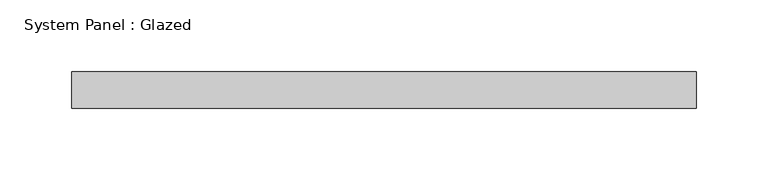
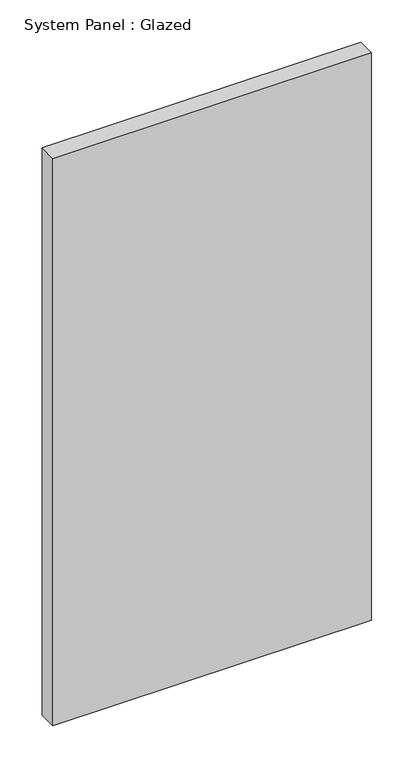
"""IFC4 building model written with IfcOpenShell, lengths in millimetres: plate geometry, System Panel : Glazed."""

from ifc_helpers import new_model, si_unit, origin, origin_with_axes, place, context, project, spatial, polyline, outline, extrude, source, transform, mapped, element, save


def system_panel_glazed_eab43fe1(model_context):
    return source(origin(), model_context, "Body", "SweptSolid", [
        extrude(outline(polyline([(217.839047, 19.05), (-217.839047, 19.05), (-217.839047, 44.45), (217.839047, 44.45), (217.839047, 19.05)])), origin_with_axes(), (0.0, 0.0, 1.0), 819.15),
    ])


if __name__ == "__main__":
    model = new_model("IFC4")
    model_context = context("Model", 3, world=origin())
    ifc_project = project(units=[si_unit("LENGTHUNIT", "METRE", prefix="MILLI")], contexts=[model_context])
    site = spatial("IfcSite", under=ifc_project)
    building = spatial("IfcBuilding", under=site)
    placement = place(None, origin())
    system_panel_glazed_shape = system_panel_glazed_eab43fe1(model_context)
    element("IfcPlate", 1, ObjectType="System Panel : Glazed", at=placement, inside=building, context=model_context, shape_type="MappedRepresentation", body=[
        mapped(system_panel_glazed_shape, transform((0.0, 0.0, 0.0), x_axis=(1.0, 0.0, 0.0), y_axis=(0.0, 1.0, 0.0), z_axis=(0.0, 0.0, 1.0))),
    ])
    save(model, "model.ifc")

# Revit data of these elements
# Element 1 (IfcPlate, "System Panel : Glazed")
#   Materials on its faces: "Glass"
# Materials
#   "Glass": class "Glass", colour RGB 0 128 192, transparency 0.75
